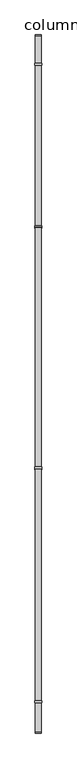
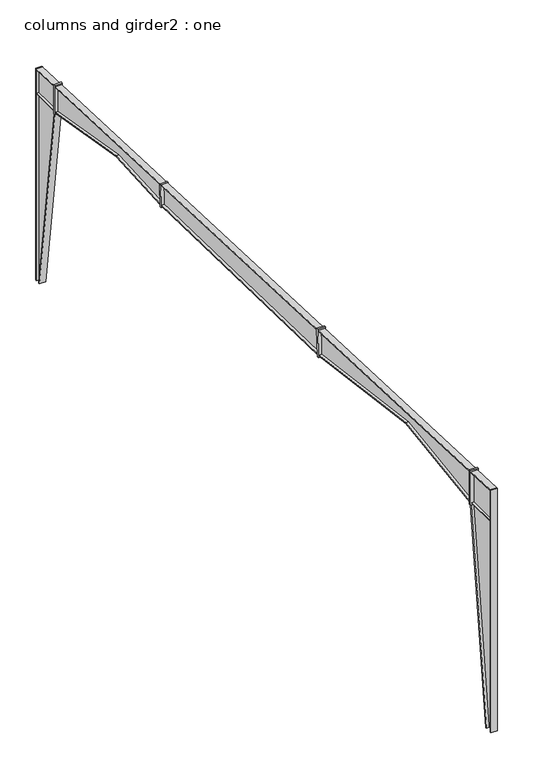
"""IFC4 building model written with IfcOpenShell, lengths in millimetres: beam geometry, columns and girder2 : one."""

import ifcopenshell
import ifcopenshell.guid

model = None  # the IFC model being written
_history = None  # IfcOwnerHistory: only IFC2X3 demands one
_inside = {}  # id of a spatial element -> (the spatial element, [elements in it])
_under = {}  # id of a project, library or spatial element -> (it, [spatial elements below it])
_declared = {}  # id of a project -> (the project, [libraries it declares])
_typed = {}  # id of a type object -> (the type object, [elements of that type])
_made_of = {}  # id of a material, layer set ... -> (it, [elements and type objects made of it])


def new_model(schema):
    """Start an empty IFC model of exactly this schema.

    Asked for "IFC4X3", IfcOpenShell would pick the latest addendum, in which some entities
    have other attributes; the version numbers below select the first issue.
    IFC2X3 requires an IfcOwnerHistory on every rooted entity: one is made here for all.
    """
    global model, _history
    if schema == "IFC4X3":
        model = ifcopenshell.file(schema_version=(4, 3, 0, 0))
    else:
        model = ifcopenshell.file(schema=schema)
    _inside.clear()
    _under.clear()
    _declared.clear()
    _typed.clear()
    _made_of.clear()
    _history = None
    if model.schema == "IFC2X3":
        org = make("IfcOrganization", Name="unknown")
        user = make(
            "IfcPersonAndOrganization",
            ThePerson=make("IfcPerson", FamilyName="unknown"),
            TheOrganization=org,
        )
        app = make(
            "IfcApplication",
            ApplicationDeveloper=org,
            Version="unknown",
            ApplicationFullName="unknown",
            ApplicationIdentifier="unknown",
        )
        _history = make(
            "IfcOwnerHistory",
            OwningUser=user,
            OwningApplication=app,
            ChangeAction="ADDED",
            CreationDate=0,
        )
    return model


def make(cls, **values):
    """One entity of the class cls with the attributes given. An attribute that is None is left unset."""
    return model.create_entity(
        cls, **{name: value for name, value in values.items() if value is not None}
    )


def rooted(cls, **values):
    """An entity with a GlobalId (a new one), such as an element, a storey or a relation."""
    return make(cls, GlobalId=ifcopenshell.guid.new(), OwnerHistory=_history, **values)


def si_unit(unit_type, name, prefix=None):
    """IfcSIUnit, for example si_unit("LENGTHUNIT", "METRE", prefix="MILLI")."""
    return make("IfcSIUnit", UnitType=unit_type, Prefix=prefix, Name=name)


def assignment(units):
    """IfcUnitAssignment: the units of a project."""
    return None if units is None else make("IfcUnitAssignment", Units=units)


def point(xyz):
    """IfcCartesianPoint."""
    return None if xyz is None else make("IfcCartesianPoint", Coordinates=xyz)


def direction(xyz):
    """IfcDirection."""
    return None if xyz is None else make("IfcDirection", DirectionRatios=xyz)


def frame(location, z_axis=None, x_axis=None):
    """IfcAxis2Placement3D, a coordinate frame: its origin and axes. An axis left out is left unset."""
    return make(
        "IfcAxis2Placement3D",
        Location=point(location),
        Axis=direction(z_axis),
        RefDirection=direction(x_axis),
    )


def origin():
    """The frame at (0, 0, 0) with its axes left unset."""
    return frame((0.0, 0.0, 0.0))


def place(relative_to, where):
    """IfcLocalPlacement: puts the frame where relative to a parent placement (None: the world)."""
    return make(
        "IfcLocalPlacement", PlacementRelTo=relative_to, RelativePlacement=where
    )


def context(
    kind, dimensions, precision=None, world=None, true_north=None, identifier=None
):
    """IfcGeometricRepresentationContext, for example the 3D "Model" context."""
    return make(
        "IfcGeometricRepresentationContext",
        ContextIdentifier=identifier,
        ContextType=kind,
        CoordinateSpaceDimension=dimensions,
        Precision=precision,
        WorldCoordinateSystem=world,
        TrueNorth=true_north,
    )


def project(units=None, contexts=None):
    """IfcProject with its units and contexts."""
    return rooted(
        "IfcProject",
        Name="project",
        RepresentationContexts=contexts,
        UnitsInContext=assignment(units),
    )


def spatial(cls, under=None, at=None, **own):
    """A site, building, storey or space (cls), placed at a placement, below another one or the project."""
    s = rooted(cls, ObjectPlacement=at, **own)
    if under is not None:
        _under.setdefault(under.id(), (under, []))[1].append(s)
    return s


def polyline(points):
    """IfcPolyline through the points."""
    return make("IfcPolyline", Points=[point(p) for p in points])


def outline(outer, holes=None, kind="AREA"):
    """IfcArbitraryClosedProfileDef: a profile drawn as a closed curve; with holes, ...WithVoids."""
    if holes is None:
        return make("IfcArbitraryClosedProfileDef", ProfileType=kind, OuterCurve=outer)
    return make(
        "IfcArbitraryProfileDefWithVoids",
        ProfileType=kind,
        OuterCurve=outer,
        InnerCurves=holes,
    )


def extrude(swept, where, along, depth):
    """IfcExtrudedAreaSolid: the profile swept, set in the frame where, extruded along a direction by depth."""
    return make(
        "IfcExtrudedAreaSolid",
        SweptArea=swept,
        Position=where,
        ExtrudedDirection=direction(along),
        Depth=depth,
    )


def shape(context_of_items, identifier, shape_type, items):
    """IfcShapeRepresentation: the items that make up one representation, for example the "Body"."""
    return make(
        "IfcShapeRepresentation",
        ContextOfItems=context_of_items,
        RepresentationIdentifier=identifier,
        RepresentationType=shape_type,
        Items=items,
    )


def source(mapping_origin, context_of_items, identifier, shape_type, items):
    """IfcRepresentationMap: a shape defined once, which mapped items show again and again."""
    return make(
        "IfcRepresentationMap",
        MappingOrigin=mapping_origin,
        MappedRepresentation=shape(context_of_items, identifier, shape_type, items),
    )


def transform(
    local_origin,
    x_axis=None,
    y_axis=None,
    z_axis=None,
    scale=None,
    scale2=None,
    scale3=None,
    uniform=True,
):
    """IfcCartesianTransformationOperator3D, or its non-uniform kind. x_axis, y_axis, z_axis: its Axis1, 2, 3."""
    if uniform:
        return make(
            "IfcCartesianTransformationOperator3D",
            Axis1=direction(x_axis),
            Axis2=direction(y_axis),
            LocalOrigin=point(local_origin),
            Scale=scale,
            Axis3=direction(z_axis),
        )
    return make(
        "IfcCartesianTransformationOperator3DnonUniform",
        Axis1=direction(x_axis),
        Axis2=direction(y_axis),
        LocalOrigin=point(local_origin),
        Scale=scale,
        Axis3=direction(z_axis),
        Scale2=scale2,
        Scale3=scale3,
    )


def mapped(mapping_source, mapping_target):
    """IfcMappedItem: shows the shape of a source again, moved by a transform."""
    return make(
        "IfcMappedItem", MappingSource=mapping_source, MappingTarget=mapping_target
    )


def made_of(thing, what):
    """Note that an element or type object is made of a material, layer set ...; save() writes the relation."""
    if what is not None:
        _made_of.setdefault(what.id(), (what, []))[1].append(thing)
    return thing


def element(
    cls,
    number,
    at=None,
    inside=None,
    cuts=None,
    type_object=None,
    material=None,
    context=None,
    identifier="Body",
    shape_type=None,
    held_by="IfcProductDefinitionShape",
    body=None,
    shapes=None,
    **own,
):
    """One element of the class cls, such as IfcWall. Its Tag is "e" and its number.

    at: its placement. inside: the storey or other place that contains it. cuts: it is an
    opening in that element (IfcRelVoidsElement). A single representation is given by context,
    identifier, shape_type and body (its items); several are given by shapes. held_by: the class
    of the entity that holds the representations. save() writes the other relations.
    """
    e = rooted(cls, Tag="e%d" % number, ObjectPlacement=at, **own)
    if body is not None:
        shapes = [shape(context, identifier, shape_type, body)]
    if shapes is not None:
        e.Representation = make(held_by, Representations=shapes)
    if inside is not None:
        _inside.setdefault(inside.id(), (inside, []))[1].append(e)
    if cuts is not None:
        rooted(
            "IfcRelVoidsElement", RelatingBuildingElement=cuts, RelatedOpeningElement=e
        )
    if type_object is not None:
        _typed.setdefault(type_object.id(), (type_object, []))[1].append(e)
    return made_of(e, material)


def aggregate(whole, parts):
    """IfcRelAggregates: a whole, such as a stair, and the parts it consists of."""
    return rooted("IfcRelAggregates", RelatingObject=whole, RelatedObjects=parts)


def save(model, path):
    """Write the relations noted so far, then the file.

    IfcRelAggregates (storeys below a building ...), IfcRelContainedInSpatialStructure (elements
    in a storey), IfcRelDefinesByType, IfcRelAssociatesMaterial and IfcRelDeclares: one each for
    every whole, place, type object, material and project.
    """
    for whole, parts in _under.values():
        aggregate(whole, parts)
    for where, things in _inside.values():
        rooted(
            "IfcRelContainedInSpatialStructure",
            RelatedElements=things,
            RelatingStructure=where,
        )
    for kind, things in _typed.values():
        rooted("IfcRelDefinesByType", RelatedObjects=things, RelatingType=kind)
    for what, things in _made_of.values():
        rooted("IfcRelAssociatesMaterial", RelatedObjects=things, RelatingMaterial=what)
    for by, libraries in _declared.values():
        rooted("IfcRelDeclares", RelatingContext=by, RelatedDefinitions=libraries)
    model.write(path)


def columns_and_girder2_one_f218e51f(model_context):
    return source(origin(), model_context, "Body", "SweptSolid", [
        extrude(outline(polyline([(-31095.9500483, 9827.2388004), (-50.8, 8533.6646481), (-50.8, -241.300095), (-233.7880954, -241.300095), (-1295.0679827, 7552.5651473), (-5516.7604947, 8278.3956415), (-8590.6692012, 8101.4110555), (-19349.8972856, 8371.7588346), (-25325.3447249, 9154.5998473), (-29764.155629, 8521.0470733), (-30818.3171044, -241.300095), (-31095.9500483, -241.300095), (-31095.9500483, 9827.2388004)])), frame((-15.875, 0.0, 0.0), z_axis=(1.0, 0.0, 0.0), x_axis=(0.0, 1.0, 0.0)), (0.0, 0.0, 1.0), 31.75),
        extrude(outline(polyline([(-12.7, -241.300095), (-50.8, -241.300095), (-50.8, 8577.5487827), (-12.7, 8575.9613919), (-12.7, -241.300095)])), frame((-127.0, 0.0, 0.0), z_axis=(1.0, 0.0, 0.0), x_axis=(0.0, 1.0, 0.0)), (0.0, 0.0, 1.0), 254.0),
        extrude(outline(polyline([(-31134.0500483, 9872.6640393), (-31095.9500483, 9871.0765058), (-31095.9500483, -241.3001099), (-31134.0500483, -241.3001099), (-31134.0500483, 9872.6640393)])), frame((-127.0, 0.0, 0.0), z_axis=(1.0, 0.0, 0.0), x_axis=(0.0, 1.0, 0.0)), (0.0, 0.0, 1.0), 254.0),
        extrude(outline(polyline([(-1321.1519467, 7461.7389652), (-1282.7003067, 7461.7389652), (-233.7880954, -241.300095), (-272.2396872, -241.300095), (-1321.1519467, 7461.7389652)])), frame((-127.0, 0.0, 0.0), z_axis=(1.0, 0.0, 0.0), x_axis=(0.0, 1.0, 0.0)), (0.0, 0.0, 1.0), 254.0),
        extrude(outline(polyline([(-29775.1493619, 8429.665528), (-29736.7735028, 8429.665528), (-30779.9412471, -241.3001099), (-30818.3171062, -241.3001099), (-29775.1493619, 8429.665528)])), frame((-127.0, 0.0, 0.0), z_axis=(1.0, 0.0, 0.0), x_axis=(0.0, 1.0, 0.0)), (0.0, 0.0, 1.0), 254.0),
        extrude(outline(polyline([(101.6, -50.8), (101.6, -1282.7003067), (-101.6, -1282.7003067), (-101.6, -50.8), (101.6, -50.8)])), frame((0.0, 0.0, 7531.5882052), z_axis=(0.0, 0.0, 1.0), x_axis=(1.0, 0.0, 0.0)), (0.0, 0.0, 1.0), 25.40001),
        extrude(outline(polyline([(101.6, -29775.1493619), (101.6, -31095.9500483), (-101.6, -31095.9500483), (-101.6, -29775.1493619), (101.6, -29775.1493619)])), frame((0.0, 0.0, 8499.5163175), z_axis=(0.0, 0.0, 1.0), x_axis=(1.0, 0.0, 0.0)), (0.0, 0.0, 1.0), 25.40001),
        extrude(outline(polyline([(152.4, -29698.9493319), (152.4, -29775.1493619), (-152.4, -29775.1493619), (-152.4, -29698.9493319), (152.4, -29698.9493319)])), frame((0.0, 0.0, 8429.665528), z_axis=(0.0, 0.0, 1.0), x_axis=(1.0, 0.0, 0.0)), (0.0, 0.0, 1.0), 1436.1811065),
        extrude(outline(polyline([(0.0, -76.1994087), (0.0, 0.0), (304.8, 0.0), (304.8, -76.1994087), (0.0, -76.1994087)])), frame((152.4, -8632.7059976, 8007.830038), z_axis=(0.0, 0.041631065796131184, 0.9991330513803847), x_axis=(-1.0, 0.0, 0.0)), (0.0, 0.0, 1.0), 920.7495558),
        extrude(outline(polyline([(152.4, -1282.7003067), (152.4, -1358.9003367), (-152.4, -1358.9003367), (-152.4, -1282.7003067), (152.4, -1282.7003067)])), frame((0.0, 0.0, 7461.7389652), z_axis=(0.0, 0.0, 1.0), x_axis=(1.0, 0.0, 0.0)), (0.0, 0.0, 1.0), 1220.092654),
        extrude(outline(polyline([(-19391.9310414, 8278.177811), (-19343.817682, 9432.8760068), (-19267.6827523, 9429.7041043), (-19315.7961116, 8275.0059086), (-19391.9310414, 8278.177811)])), frame((-152.4, 0.0, 0.0), z_axis=(1.0, 0.0, 0.0), x_axis=(0.0, 1.0, 0.0)), (0.0, 0.0, 1.0), 304.8),
        extrude(outline(polyline([(-31134.0500483, 9866.9346266), (-12.7, 8570.2115212), (-12.7, 8532.0771159), (-31134.0500483, 9828.8263326), (-31134.0500483, 9866.9346266)])), frame((-127.0, 0.0, 0.0), z_axis=(1.0, 0.0, 0.0), x_axis=(0.0, 1.0, 0.0)), (0.0, 0.0, 1.0), 254.0),
        extrude(outline(polyline([(-29698.9493319, 8491.8679427), (-29698.9493319, 8530.3539871), (-25325.3447249, 9154.5998473), (-19349.8972856, 8371.7588346), (-8590.6692012, 8101.4110555), (-5516.7604947, 8278.3956415), (-1358.9003367, 7563.5397668), (-1358.9003367, 7524.880088), (-5518.9211974, 8240.108022), (-8590.0491198, 8063.283485), (-19352.8597593, 8333.7212968), (-25325.1199348, 9116.1456038), (-29698.9493319, 8491.8679427)])), frame((-127.0, 0.0, 0.0), z_axis=(1.0, 0.0, 0.0), x_axis=(0.0, 1.0, 0.0)), (0.0, 0.0, 1.0), 254.0),
    ])


if __name__ == "__main__":
    model = new_model("IFC4")
    model_context = context("Model", 3, world=origin())
    ifc_project = project(units=[si_unit("LENGTHUNIT", "METRE", prefix="MILLI")], contexts=[model_context])
    site = spatial("IfcSite", under=ifc_project)
    building = spatial("IfcBuilding", under=site)
    placement = place(None, origin())
    columns_and_girder2_one_shape = columns_and_girder2_one_f218e51f(model_context)
    element("IfcBeam", 1, ObjectType="columns and girder2 : one", at=placement, inside=building, context=model_context, shape_type="MappedRepresentation", body=[
        mapped(columns_and_girder2_one_shape, transform((0.0, 0.0, 0.0), x_axis=(1.0, 0.0, 0.0), y_axis=(0.0, 1.0, 0.0), z_axis=(0.0, 0.0, 1.0))),
    ])
    save(model, "model.ifc")

# Revit data of these elements
# Type "columns and girder2 : one"
#   web thickness = 0' - 1 1/4"
#   stiffeners = 0' - 8"
#   plate width = 1' - 0"
#   flange width = 0' - 10"
#   Structural Material [instance default] = none
# Element 1 (IfcBeam, "columns and girder2 : one")
#   Structural Material = STRUCTURAL STEEL - SEE STRUCT. DWGS
#   Materials on its faces: "STRUCTURAL STEEL - SEE STRUCT. DWGS"
# Materials
#   "STRUCTURAL STEEL - SEE STRUCT. DWGS": class "Metal", colour RGB 137 146 153, transparency 0, Description = "Steel, mill finish", Cost = 0
